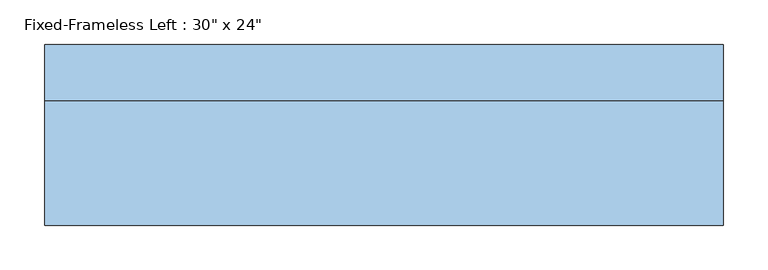
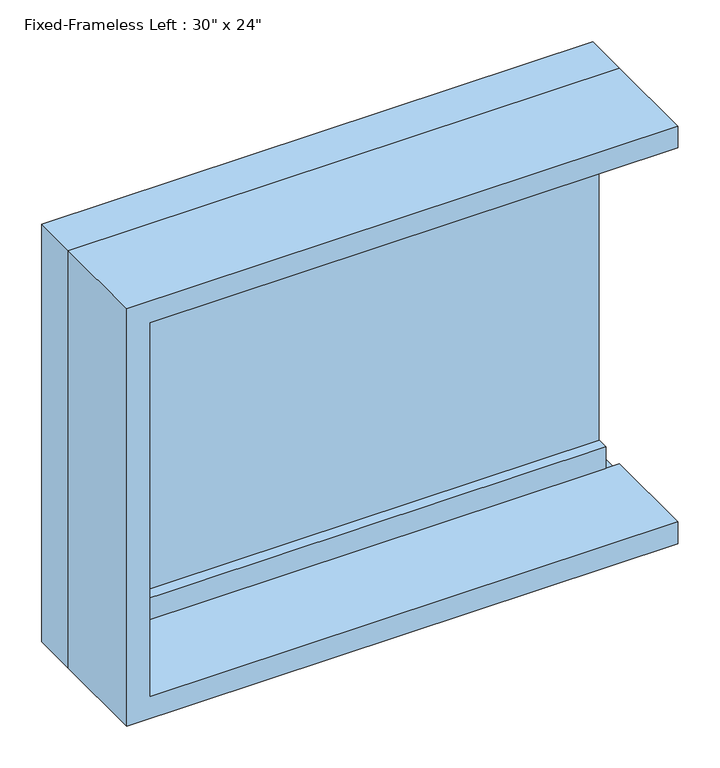
"""IFC4 building model written with IfcOpenShell, lengths in millimetres: window geometry."""

import ifcopenshell
import ifcopenshell.guid

model = None  # the IFC model being written
_history = None  # IfcOwnerHistory: only IFC2X3 demands one
_inside = {}  # id of a spatial element -> (the spatial element, [elements in it])
_under = {}  # id of a project, library or spatial element -> (it, [spatial elements below it])
_declared = {}  # id of a project -> (the project, [libraries it declares])
_typed = {}  # id of a type object -> (the type object, [elements of that type])
_made_of = {}  # id of a material, layer set ... -> (it, [elements and type objects made of it])


def new_model(schema):
    """Start an empty IFC model of exactly this schema.

    Asked for "IFC4X3", IfcOpenShell would pick the latest addendum, in which some entities
    have other attributes; the version numbers below select the first issue.
    IFC2X3 requires an IfcOwnerHistory on every rooted entity: one is made here for all.
    """
    global model, _history
    if schema == "IFC4X3":
        model = ifcopenshell.file(schema_version=(4, 3, 0, 0))
    else:
        model = ifcopenshell.file(schema=schema)
    _inside.clear()
    _under.clear()
    _declared.clear()
    _typed.clear()
    _made_of.clear()
    _history = None
    if model.schema == "IFC2X3":
        org = make("IfcOrganization", Name="unknown")
        user = make(
            "IfcPersonAndOrganization",
            ThePerson=make("IfcPerson", FamilyName="unknown"),
            TheOrganization=org,
        )
        app = make(
            "IfcApplication",
            ApplicationDeveloper=org,
            Version="unknown",
            ApplicationFullName="unknown",
            ApplicationIdentifier="unknown",
        )
        _history = make(
            "IfcOwnerHistory",
            OwningUser=user,
            OwningApplication=app,
            ChangeAction="ADDED",
            CreationDate=0,
        )
    return model


def make(cls, **values):
    """One entity of the class cls with the attributes given. An attribute that is None is left unset."""
    return model.create_entity(
        cls, **{name: value for name, value in values.items() if value is not None}
    )


def rooted(cls, **values):
    """An entity with a GlobalId (a new one), such as an element, a storey or a relation."""
    return make(cls, GlobalId=ifcopenshell.guid.new(), OwnerHistory=_history, **values)


def si_unit(unit_type, name, prefix=None):
    """IfcSIUnit, for example si_unit("LENGTHUNIT", "METRE", prefix="MILLI")."""
    return make("IfcSIUnit", UnitType=unit_type, Prefix=prefix, Name=name)


def assignment(units):
    """IfcUnitAssignment: the units of a project."""
    return None if units is None else make("IfcUnitAssignment", Units=units)


def point(xyz):
    """IfcCartesianPoint."""
    return None if xyz is None else make("IfcCartesianPoint", Coordinates=xyz)


def direction(xyz):
    """IfcDirection."""
    return None if xyz is None else make("IfcDirection", DirectionRatios=xyz)


def frame(location, z_axis=None, x_axis=None):
    """IfcAxis2Placement3D, a coordinate frame: its origin and axes. An axis left out is left unset."""
    return make(
        "IfcAxis2Placement3D",
        Location=point(location),
        Axis=direction(z_axis),
        RefDirection=direction(x_axis),
    )


def origin():
    """The frame at (0, 0, 0) with its axes left unset."""
    return frame((0.0, 0.0, 0.0))


def place(relative_to, where):
    """IfcLocalPlacement: puts the frame where relative to a parent placement (None: the world)."""
    return make(
        "IfcLocalPlacement", PlacementRelTo=relative_to, RelativePlacement=where
    )


def context(
    kind, dimensions, precision=None, world=None, true_north=None, identifier=None
):
    """IfcGeometricRepresentationContext, for example the 3D "Model" context."""
    return make(
        "IfcGeometricRepresentationContext",
        ContextIdentifier=identifier,
        ContextType=kind,
        CoordinateSpaceDimension=dimensions,
        Precision=precision,
        WorldCoordinateSystem=world,
        TrueNorth=true_north,
    )


def project(units=None, contexts=None):
    """IfcProject with its units and contexts."""
    return rooted(
        "IfcProject",
        Name="project",
        RepresentationContexts=contexts,
        UnitsInContext=assignment(units),
    )


def spatial(cls, under=None, at=None, **own):
    """A site, building, storey or space (cls), placed at a placement, below another one or the project."""
    s = rooted(cls, ObjectPlacement=at, **own)
    if under is not None:
        _under.setdefault(under.id(), (under, []))[1].append(s)
    return s


def polyline(points):
    """IfcPolyline through the points."""
    return make("IfcPolyline", Points=[point(p) for p in points])


def outline(outer, holes=None, kind="AREA"):
    """IfcArbitraryClosedProfileDef: a profile drawn as a closed curve; with holes, ...WithVoids."""
    if holes is None:
        return make("IfcArbitraryClosedProfileDef", ProfileType=kind, OuterCurve=outer)
    return make(
        "IfcArbitraryProfileDefWithVoids",
        ProfileType=kind,
        OuterCurve=outer,
        InnerCurves=holes,
    )


def extrude(swept, where, along, depth):
    """IfcExtrudedAreaSolid: the profile swept, set in the frame where, extruded along a direction by depth."""
    return make(
        "IfcExtrudedAreaSolid",
        SweptArea=swept,
        Position=where,
        ExtrudedDirection=direction(along),
        Depth=depth,
    )


def shape(context_of_items, identifier, shape_type, items):
    """IfcShapeRepresentation: the items that make up one representation, for example the "Body"."""
    return make(
        "IfcShapeRepresentation",
        ContextOfItems=context_of_items,
        RepresentationIdentifier=identifier,
        RepresentationType=shape_type,
        Items=items,
    )


def source(mapping_origin, context_of_items, identifier, shape_type, items):
    """IfcRepresentationMap: a shape defined once, which mapped items show again and again."""
    return make(
        "IfcRepresentationMap",
        MappingOrigin=mapping_origin,
        MappedRepresentation=shape(context_of_items, identifier, shape_type, items),
    )


def transform(
    local_origin,
    x_axis=None,
    y_axis=None,
    z_axis=None,
    scale=None,
    scale2=None,
    scale3=None,
    uniform=True,
):
    """IfcCartesianTransformationOperator3D, or its non-uniform kind. x_axis, y_axis, z_axis: its Axis1, 2, 3."""
    if uniform:
        return make(
            "IfcCartesianTransformationOperator3D",
            Axis1=direction(x_axis),
            Axis2=direction(y_axis),
            LocalOrigin=point(local_origin),
            Scale=scale,
            Axis3=direction(z_axis),
        )
    return make(
        "IfcCartesianTransformationOperator3DnonUniform",
        Axis1=direction(x_axis),
        Axis2=direction(y_axis),
        LocalOrigin=point(local_origin),
        Scale=scale,
        Axis3=direction(z_axis),
        Scale2=scale2,
        Scale3=scale3,
    )


def mapped(mapping_source, mapping_target):
    """IfcMappedItem: shows the shape of a source again, moved by a transform."""
    return make(
        "IfcMappedItem", MappingSource=mapping_source, MappingTarget=mapping_target
    )


def made_of(thing, what):
    """Note that an element or type object is made of a material, layer set ...; save() writes the relation."""
    if what is not None:
        _made_of.setdefault(what.id(), (what, []))[1].append(thing)
    return thing


def element(
    cls,
    number,
    at=None,
    inside=None,
    cuts=None,
    type_object=None,
    material=None,
    context=None,
    identifier="Body",
    shape_type=None,
    held_by="IfcProductDefinitionShape",
    body=None,
    shapes=None,
    **own,
):
    """One element of the class cls, such as IfcWall. Its Tag is "e" and its number.

    at: its placement. inside: the storey or other place that contains it. cuts: it is an
    opening in that element (IfcRelVoidsElement). A single representation is given by context,
    identifier, shape_type and body (its items); several are given by shapes. held_by: the class
    of the entity that holds the representations. save() writes the other relations.
    """
    e = rooted(cls, Tag="e%d" % number, ObjectPlacement=at, **own)
    if body is not None:
        shapes = [shape(context, identifier, shape_type, body)]
    if shapes is not None:
        e.Representation = make(held_by, Representations=shapes)
    if inside is not None:
        _inside.setdefault(inside.id(), (inside, []))[1].append(e)
    if cuts is not None:
        rooted(
            "IfcRelVoidsElement", RelatingBuildingElement=cuts, RelatedOpeningElement=e
        )
    if type_object is not None:
        _typed.setdefault(type_object.id(), (type_object, []))[1].append(e)
    return made_of(e, material)


def aggregate(whole, parts):
    """IfcRelAggregates: a whole, such as a stair, and the parts it consists of."""
    return rooted("IfcRelAggregates", RelatingObject=whole, RelatedObjects=parts)


def save(model, path):
    """Write the relations noted so far, then the file.

    IfcRelAggregates (storeys below a building ...), IfcRelContainedInSpatialStructure (elements
    in a storey), IfcRelDefinesByType, IfcRelAssociatesMaterial and IfcRelDeclares: one each for
    every whole, place, type object, material and project.
    """
    for whole, parts in _under.values():
        aggregate(whole, parts)
    for where, things in _inside.values():
        rooted(
            "IfcRelContainedInSpatialStructure",
            RelatedElements=things,
            RelatingStructure=where,
        )
    for kind, things in _typed.values():
        rooted("IfcRelDefinesByType", RelatedObjects=things, RelatingType=kind)
    for what, things in _made_of.values():
        rooted("IfcRelAssociatesMaterial", RelatedObjects=things, RelatingMaterial=what)
    for by, libraries in _declared.values():
        rooted("IfcRelDeclares", RelatingContext=by, RelatedDefinitions=libraries)
    model.write(path)


def window_60832851(model_context):
    return source(origin(), model_context, "Body", "SweptSolid", [
        extrude(outline(polyline([(323.85, 53.975), (-355.6, 53.975), (-355.6, 66.675), (323.85, 66.675), (323.85, 53.975)])), frame((0.0, 0.0, 977.9), z_axis=(0.0, 0.0, 1.0), x_axis=(1.0, 0.0, 0.0)), (0.0, 0.0, 1.0), 482.6),
        extrude(outline(polyline([(1504.95, -400.05), (933.45, -400.05), (933.45, 323.85), (977.9, 323.85), (977.9, -355.6), (1460.5, -355.6), (1460.5, 323.85), (1504.95, 323.85), (1504.95, -400.05)])), frame((0.0, 38.1, 0.0), z_axis=(0.0, 1.0, 0.0), x_axis=(0.0, 0.0, 1.0)), (0.0, 0.0, 1.0), 44.45),
        extrude(outline(polyline([(1524.0, -419.1), (914.4, -419.1), (914.4, 342.9), (946.15, 342.9), (946.15, -387.35), (1492.25, -387.35), (1492.25, 342.9), (1524.0, 342.9), (1524.0, -419.1)])), frame((0.0, -101.6, 0.0), z_axis=(0.0, 1.0, 0.0), x_axis=(0.0, 0.0, 1.0)), (0.0, 0.0, 1.0), 139.7),
        extrude(outline(polyline([(1524.0, 342.9), (1524.0, -419.1), (914.4, -419.1), (914.4, 342.9), (933.45, 342.9), (933.45, -400.05), (1504.95, -400.05), (1504.95, 342.9), (1524.0, 342.9)])), frame((0.0, 38.1, 0.0), z_axis=(0.0, 1.0, 0.0), x_axis=(0.0, 0.0, 1.0)), (0.0, 0.0, 1.0), 63.5),
    ])


if __name__ == "__main__":
    model = new_model("IFC4")
    model_context = context("Model", 3, world=origin())
    ifc_project = project(units=[si_unit("LENGTHUNIT", "METRE", prefix="MILLI")], contexts=[model_context])
    site = spatial("IfcSite", under=ifc_project)
    building = spatial("IfcBuilding", under=site)
    placement = place(None, origin())
    window_shape = window_60832851(model_context)
    element("IfcWindow", 1, ObjectType="Fixed-Frameless Left : 30\" x 24\"", at=placement, inside=building, context=model_context, shape_type="MappedRepresentation", body=[
        mapped(window_shape, transform((0.0, 0.0, 0.0), x_axis=(1.0, 0.0, 0.0), y_axis=(0.0, 1.0, 0.0), z_axis=(0.0, 0.0, 1.0))),
    ])
    save(model, "model.ifc")

# Revit data of these elements
# Type "Fixed-Frameless Left : 30\" x 24\""
#   Type Mark = "77"
#   Assembly Code = "B2020100"
#   Height = 2' - 0"
#   Default Sill Height = 3' - 0"
#   Width = 2' - 6"
#   Window Inset = 0' - 0 3/4"
#   Glass Pane Material = Glass
#   Sash Material = Sash
#   Wall Closure = (empty or 0)
# Element 1 (IfcWindow, "Fixed-Frameless Left : 30\" x 24\"")
#   Materials on its faces: "Sash", "Glass"
# Materials
#   "Glass": class "Glass", colour RGB 0 128 192, transparency 0.75
#   "Sash": class "Wood", colour RGB 224 178 126, transparency 0
